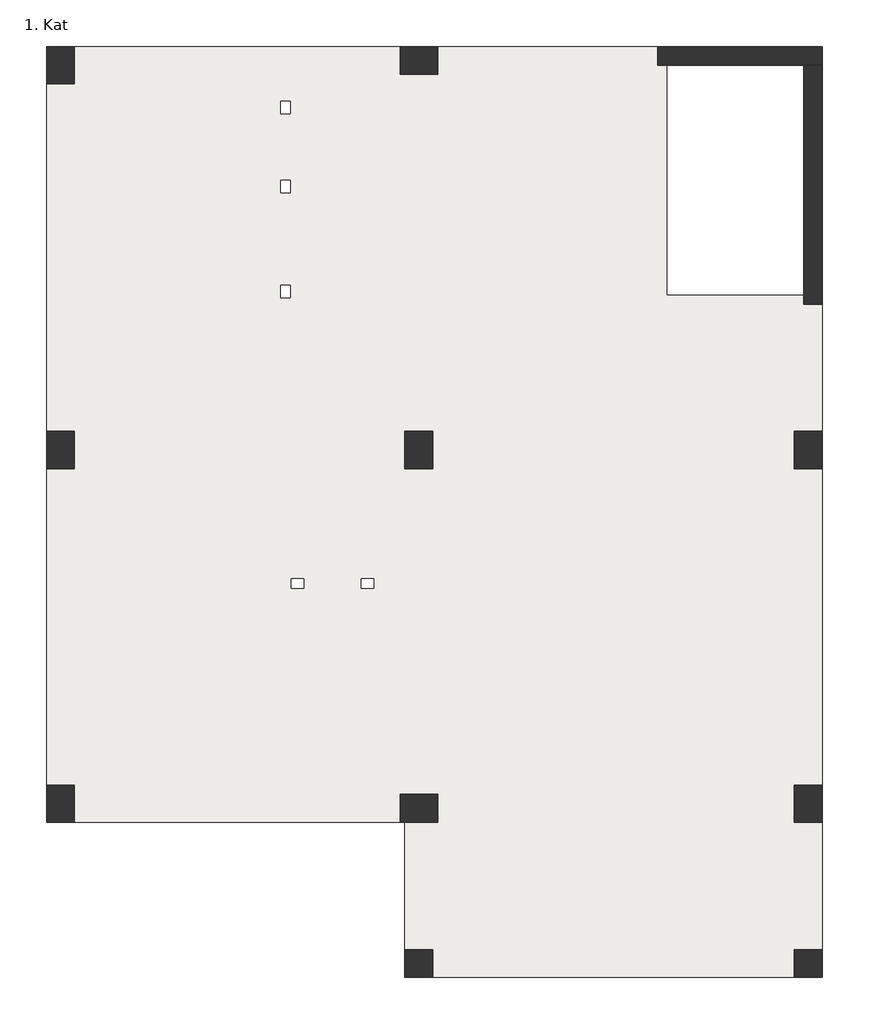
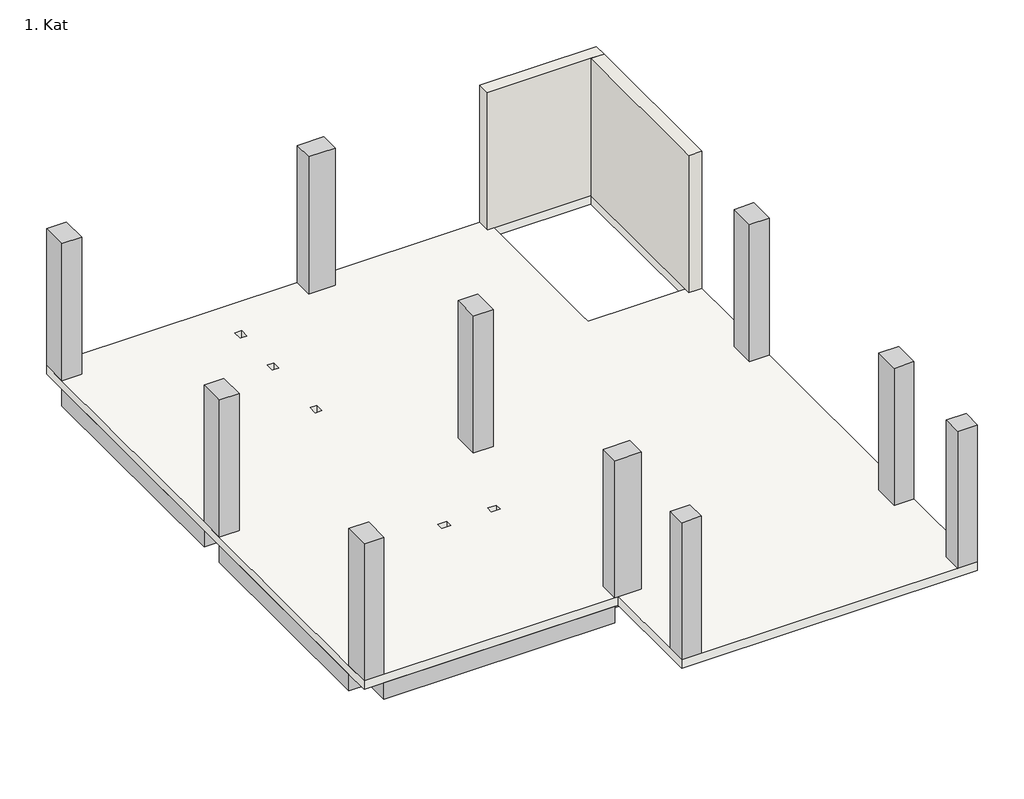
# One storey: 12 beams, 10 columns, 2 walls, 1 slab.
"""IFC4 building model written with IfcOpenShell, lengths in millimetres."""

from ifc_helpers import new_model, si_unit, frame, origin, place, context, project, spatial, polyline, outline, extrude, faceted_brep, element, save

model = new_model("IFC4")

# Units and contexts
model_context = context("Model", 3, world=origin())
ifc_project = project(units=[si_unit("LENGTHUNIT", "METRE", prefix="MILLI")], contexts=[model_context])

# Site, building, storey
site = spatial("IfcSite", under=ifc_project)
building = spatial("IfcBuilding", under=site)
storey = spatial("IfcBuildingStorey", under=building, Name="1. Kat", Elevation=97280.0)

# Beams
placement = place(None, origin())
element("IfcBeam", 1, ObjectType="M_Concrete-Rectangular Beam : 300 x 600mm", at=placement, inside=storey, context=model_context, shape_type="SweptSolid", body=[
    extrude(outline(polyline([(-8879.0485128, 8478.2904426), (-8879.0485128, 8778.2904426), (-5329.0485128, 8778.2904426), (-5329.0485128, 8478.2904426), (-8879.0485128, 8478.2904426)])), frame((0.0, 0.0, 96680.0), z_axis=(0.0, 0.0, 1.0), x_axis=(1.0, 0.0, 0.0)), (0.0, 0.0, 1.0), 400.0),
])
element("IfcBeam", 2, ObjectType="M_Concrete-Rectangular Beam : 300 x 600mm", at=placement, inside=storey, context=model_context, shape_type="SweptSolid", body=[
    extrude(outline(polyline([(-2679.0485128, 2578.2904426), (-2979.0485128, 2578.2904426), (-2979.0485128, 4628.2904426), (-2679.0485128, 4628.2904426), (-2679.0485128, 2578.2904426)])), frame((0.0, 0.0, 96680.0), z_axis=(0.0, 0.0, 1.0), x_axis=(1.0, 0.0, 0.0)), (0.0, 0.0, 1.0), 400.0),
])
element("IfcBeam", 3, ObjectType="M_Concrete-Rectangular Beam : 450 x 600mm", at=placement, inside=storey, context=model_context, shape_type="SweptSolid", body=[
    extrude(outline(polyline([(-8954.0485128, 1978.2904426), (-8954.0485128, -3271.7095574), (-9404.0485128, -3271.7095574), (-9404.0485128, 1978.2904426), (-8954.0485128, 1978.2904426)])), frame((0.0, 0.0, 96680.0), z_axis=(0.0, 0.0, 1.0), x_axis=(1.0, 0.0, 0.0)), (0.0, 0.0, 1.0), 400.0),
])
element("IfcBeam", 4, ObjectType="M_Concrete-Rectangular Beam : 450 x 600mm", at=placement, inside=storey, context=model_context, shape_type="SweptSolid", body=[
    extrude(outline(polyline([(-8954.0485128, 8328.2904426), (-8954.0485128, 2578.2904426), (-9404.0485128, 2578.2904426), (-9404.0485128, 8328.2904426), (-8954.0485128, 8328.2904426)])), frame((0.0, 0.0, 96680.0), z_axis=(0.0, 0.0, 1.0), x_axis=(1.0, 0.0, 0.0)), (0.0, 0.0, 1.0), 400.0),
])
element("IfcBeam", 5, ObjectType="M_Concrete-Rectangular Beam : 450 x 600mm", at=placement, inside=storey, context=model_context, shape_type="SweptSolid", body=[
    extrude(outline(polyline([(-9404.0485128, 2053.2904426), (-14729.0485128, 2053.2904426), (-14729.0485128, 2503.2904426), (-9404.0485128, 2503.2904426), (-9404.0485128, 2053.2904426)])), frame((0.0, 0.0, 96680.0), z_axis=(0.0, 0.0, 1.0), x_axis=(1.0, 0.0, 0.0)), (0.0, 0.0, 1.0), 400.0),
])
element("IfcBeam", 6, ObjectType="M_Concrete-Rectangular Beam : 450 x 600mm", at=placement, inside=storey, context=model_context, shape_type="SweptSolid", body=[
    extrude(outline(polyline([(-3129.0485128, 2053.2904426), (-8954.0485128, 2053.2904426), (-8954.0485128, 2503.2904426), (-3129.0485128, 2503.2904426), (-3129.0485128, 2053.2904426)])), frame((0.0, 0.0, 96680.0), z_axis=(0.0, 0.0, 1.0), x_axis=(1.0, 0.0, 0.0)), (0.0, 0.0, 1.0), 400.0),
])
element("IfcBeam", 7, ObjectType="M_Concrete-Rectangular Beam : 450 x 600mm", at=placement, inside=storey, context=model_context, shape_type="SweptSolid", body=[
    extrude(outline(polyline([(-9479.0485128, 8778.2904426), (-9479.0485128, 8328.2904426), (-14729.0485128, 8328.2904426), (-14729.0485128, 8778.2904426), (-9479.0485128, 8778.2904426)])), frame((0.0, 0.0, 96680.0), z_axis=(0.0, 0.0, 1.0), x_axis=(1.0, 0.0, 0.0)), (0.0, 0.0, 1.0), 400.0),
])
element("IfcBeam", 8, ObjectType="M_Concrete-Rectangular Beam : 450 x 600mm", at=placement, inside=storey, context=model_context, shape_type="SweptSolid", body=[
    extrude(outline(polyline([(-2679.0485128, -3121.7095574), (-3129.0485128, -3121.7095574), (-3129.0485128, 1978.2904426), (-2679.0485128, 1978.2904426), (-2679.0485128, -3121.7095574)])), frame((0.0, 0.0, 96680.0), z_axis=(0.0, 0.0, 1.0), x_axis=(1.0, 0.0, 0.0)), (0.0, 0.0, 1.0), 400.0),
])
element("IfcBeam", 9, ObjectType="M_Concrete-Rectangular Beam : 450 x 600mm", at=placement, inside=storey, context=model_context, shape_type="SweptSolid", body=[
    extrude(outline(polyline([(-9479.0485128, -3271.7095574), (-9479.0485128, -3721.7095574), (-14729.0485128, -3721.7095574), (-14729.0485128, -3271.7095574), (-9479.0485128, -3271.7095574)])), frame((0.0, 0.0, 96680.0), z_axis=(0.0, 0.0, 1.0), x_axis=(1.0, 0.0, 0.0)), (0.0, 0.0, 1.0), 400.0),
])
element("IfcBeam", 10, ObjectType="M_Concrete-Rectangular Beam : 450 x 600mm", at=placement, inside=storey, context=model_context, shape_type="SweptSolid", body=[
    extrude(outline(polyline([(-8879.0485128, -3721.7095574), (-8879.0485128, -3271.7095574), (-3129.0485128, -3271.7095574), (-3129.0485128, -3721.7095574), (-8879.0485128, -3721.7095574)])), frame((0.0, 0.0, 96680.0), z_axis=(0.0, 0.0, 1.0), x_axis=(1.0, 0.0, 0.0)), (0.0, 0.0, 1.0), 400.0),
])
element("IfcBeam", 11, ObjectType="M_Concrete-Rectangular Beam : 450 x 600mm", at=placement, inside=storey, context=model_context, shape_type="SweptSolid", body=[
    extrude(outline(polyline([(-14729.0485128, 2578.2904426), (-15179.0485128, 2578.2904426), (-15179.0485128, 8178.2904426), (-14729.0485128, 8178.2904426), (-14729.0485128, 2578.2904426)])), frame((0.0, 0.0, 96680.0), z_axis=(0.0, 0.0, 1.0), x_axis=(1.0, 0.0, 0.0)), (0.0, 0.0, 1.0), 400.0),
])
element("IfcBeam", 12, ObjectType="M_Concrete-Rectangular Beam : 450 x 600mm", at=placement, inside=storey, context=model_context, shape_type="SweptSolid", body=[
    extrude(outline(polyline([(-15179.0485128, 1978.2904426), (-14729.0485128, 1978.2904426), (-14729.0485128, -3121.7095574), (-15179.0485128, -3121.7095574), (-15179.0485128, 1978.2904426)])), frame((0.0, 0.0, 96680.0), z_axis=(0.0, 0.0, 1.0), x_axis=(1.0, 0.0, 0.0)), (0.0, 0.0, 1.0), 400.0),
])

# Columns
element("IfcColumn", 13, ObjectType="M_Concrete-Rectangular-Column : 450 x 450mm", at=placement, inside=storey, context=model_context, shape_type="SweptSolid", body=[
    extrude(outline(polyline([(-8954.0485128, -6221.7095574), (-9404.0485128, -6221.7095574), (-9404.0485128, -5771.7095574), (-8954.0485128, -5771.7095574), (-8954.0485128, -6221.7095574)])), frame((0.0, 0.0, 97280.0), z_axis=(0.0, 0.0, 1.0), x_axis=(1.0, 0.0, 0.0)), (0.0, 0.0, 1.0), 3300.0),
])
element("IfcColumn", 14, ObjectType="M_Concrete-Rectangular-Column : 450 x 450mm", at=placement, inside=storey, context=model_context, shape_type="SweptSolid", body=[
    extrude(outline(polyline([(-3129.0485128, -6221.7095574), (-3129.0485128, -5771.7095574), (-2679.0485128, -5771.7095574), (-2679.0485128, -6221.7095574), (-3129.0485128, -6221.7095574)])), frame((0.0, 0.0, 97280.0), z_axis=(0.0, 0.0, 1.0), x_axis=(1.0, 0.0, 0.0)), (0.0, 0.0, 1.0), 3300.0),
])
element("IfcColumn", 15, ObjectType="M_Concrete-Rectangular-Column : 450 x 600mm", at=placement, inside=storey, context=model_context, shape_type="SweptSolid", body=[
    extrude(outline(polyline([(-15179.0485128, -3721.7095574), (-15179.0485128, -3121.7095574), (-14729.0485128, -3121.7095574), (-14729.0485128, -3721.7095574), (-15179.0485128, -3721.7095574)])), frame((0.0, 0.0, 97280.0), z_axis=(0.0, 0.0, 1.0), x_axis=(1.0, 0.0, 0.0)), (0.0, 0.0, 1.0), 3300.0),
])
element("IfcColumn", 16, ObjectType="M_Concrete-Rectangular-Column : 450 x 600mm", at=placement, inside=storey, context=model_context, shape_type="SweptSolid", body=[
    extrude(outline(polyline([(-15179.0485128, 1978.2904426), (-15179.0485128, 2578.2904426), (-14729.0485128, 2578.2904426), (-14729.0485128, 1978.2904426), (-15179.0485128, 1978.2904426)])), frame((0.0, 0.0, 97280.0), z_axis=(0.0, 0.0, 1.0), x_axis=(1.0, 0.0, 0.0)), (0.0, 0.0, 1.0), 3300.0),
])
element("IfcColumn", 17, ObjectType="M_Concrete-Rectangular-Column : 450 x 600mm", at=placement, inside=storey, context=model_context, shape_type="SweptSolid", body=[
    extrude(outline(polyline([(-15179.0485128, 8178.2904426), (-15179.0485128, 8778.2904426), (-14729.0485128, 8778.2904426), (-14729.0485128, 8178.2904426), (-15179.0485128, 8178.2904426)])), frame((0.0, 0.0, 97280.0), z_axis=(0.0, 0.0, 1.0), x_axis=(1.0, 0.0, 0.0)), (0.0, 0.0, 1.0), 3300.0),
])
element("IfcColumn", 18, ObjectType="M_Concrete-Rectangular-Column : 450 x 600mm", at=placement, inside=storey, context=model_context, shape_type="Brep", body=[
    faceted_brep([(-8879.0485128, -3721.7095574, 97280.0), (-9404.0485128, -3721.7095574, 97280.0), (-9479.0485128, -3721.7095574, 97280.0), (-9479.0485128, -3271.7095574, 97280.0), (-8879.0485128, -3271.7095574, 97280.0), (-8879.0485128, -3721.7095574, 100580.0), (-9479.0485128, -3721.7095574, 100580.0), (-9479.0485128, -3271.7095574, 100580.0), (-8879.0485128, -3271.7095574, 100580.0)], [[[0, 1, 2, 3, 4]], [[2, 1, 0, 5, 6]], [[3, 2, 6, 7]], [[4, 3, 7, 8]], [[0, 4, 8, 5]], [[6, 5, 8, 7]]]),
])
element("IfcColumn", 19, ObjectType="M_Concrete-Rectangular-Column : 450 x 600mm", at=placement, inside=storey, context=model_context, shape_type="SweptSolid", body=[
    extrude(outline(polyline([(-9404.0485128, 1978.2904426), (-9404.0485128, 2578.2904426), (-8954.0485128, 2578.2904426), (-8954.0485128, 1978.2904426), (-9404.0485128, 1978.2904426)])), frame((0.0, 0.0, 97280.0), z_axis=(0.0, 0.0, 1.0), x_axis=(1.0, 0.0, 0.0)), (0.0, 0.0, 1.0), 3300.0),
])
element("IfcColumn", 20, ObjectType="M_Concrete-Rectangular-Column : 450 x 600mm", at=placement, inside=storey, context=model_context, shape_type="SweptSolid", body=[
    extrude(outline(polyline([(-8879.0485128, 8328.2904426), (-9479.0485128, 8328.2904426), (-9479.0485128, 8778.2904426), (-8879.0485128, 8778.2904426), (-8879.0485128, 8328.2904426)])), frame((0.0, 0.0, 97280.0), z_axis=(0.0, 0.0, 1.0), x_axis=(1.0, 0.0, 0.0)), (0.0, 0.0, 1.0), 3300.0),
])
element("IfcColumn", 21, ObjectType="M_Concrete-Rectangular-Column : 450 x 600mm", at=placement, inside=storey, context=model_context, shape_type="SweptSolid", body=[
    extrude(outline(polyline([(-3129.0485128, -3721.7095574), (-3129.0485128, -3121.7095574), (-2679.0485128, -3121.7095574), (-2679.0485128, -3721.7095574), (-3129.0485128, -3721.7095574)])), frame((0.0, 0.0, 97280.0), z_axis=(0.0, 0.0, 1.0), x_axis=(1.0, 0.0, 0.0)), (0.0, 0.0, 1.0), 3300.0),
])
element("IfcColumn", 22, ObjectType="M_Concrete-Rectangular-Column : 450 x 600mm", at=placement, inside=storey, context=model_context, shape_type="SweptSolid", body=[
    extrude(outline(polyline([(-3129.0485128, 1978.2904426), (-3129.0485128, 2578.2904426), (-2679.0485128, 2578.2904426), (-2679.0485128, 1978.2904426), (-3129.0485128, 1978.2904426)])), frame((0.0, 0.0, 97280.0), z_axis=(0.0, 0.0, 1.0), x_axis=(1.0, 0.0, 0.0)), (0.0, 0.0, 1.0), 3300.0),
])

# Slab
element("IfcSlab", 23, ObjectType="Generic 200mm", at=placement, inside=storey, context=model_context, shape_type="Brep", body=[
    faceted_brep([(-2679.0485128, 8778.2904426, 97080.0), (-2679.0485128, 4628.2904426, 97080.0), (-2679.0485128, 2578.2904426, 97080.0), (-2679.0485128, 1978.2904426, 97080.0), (-2679.0485128, -3121.7095574, 97080.0), (-2679.0485128, -3721.7095574, 97080.0), (-2679.0485128, -5771.7095574, 97080.0), (-2679.0485128, -6221.7095574, 97080.0), (-3129.0485128, -6221.7095574, 97080.0), (-8954.0485128, -6221.7095574, 97080.0), (-9404.0485128, -6221.7095574, 97080.0), (-9404.0485128, -5771.7095574, 97080.0), (-9404.0485128, -3721.7095574, 97080.0), (-9479.0485128, -3721.7095574, 97080.0), (-14729.0485128, -3721.7095574, 97080.0), (-15179.0485128, -3721.7095574, 97080.0), (-15179.0485128, -3121.7095574, 97080.0), (-15179.0485128, 1978.2904426, 97080.0), (-15179.0485128, 2578.2904426, 97080.0), (-15179.0485128, 8178.2904426, 97080.0), (-15179.0485128, 8778.2904426, 97080.0), (-14729.0485128, 8778.2904426, 97080.0), (-9479.0485128, 8778.2904426, 97080.0), (-8879.0485128, 8778.2904426, 97080.0), (-5329.0485128, 8778.2904426, 97080.0), (-2979.0485128, 4778.2904426, 97080.0), (-2979.0485128, 8478.2904426, 97080.0), (-5179.0485128, 8478.2904426, 97080.0), (-5179.0485128, 5253.2904426, 97080.0), (-5179.0485128, 5003.2904426, 97080.0), (-5179.0485128, 4778.2904426, 97080.0), (-4179.0485128, 4778.2904426, 97080.0), (-11404.0485128, 6624.8694152, 97080.0), (-11404.0485128, 6424.8694152, 97080.0), (-11254.0485128, 6424.8694152, 97080.0), (-11254.0485128, 6624.8694152, 97080.0), (-11404.0485128, 4933.2654426, 97080.0), (-11404.0485128, 4733.2654426, 97080.0), (-11254.0485128, 4733.2654426, 97080.0), (-11254.0485128, 4933.2654426, 97080.0), (-11404.0485128, 7898.2904426, 97080.0), (-11404.0485128, 7698.2904426, 97080.0), (-11254.0485128, 7698.2904426, 97080.0), (-11254.0485128, 7898.2904426, 97080.0), (-11232.3510299, 53.2904426, 97080.0), (-11032.3510299, 53.2904426, 97080.0), (-11032.3510299, 203.2904426, 97080.0), (-11232.3510299, 203.2904426, 97080.0), (-10104.0485128, 53.2904426, 97080.0), (-9904.0485128, 53.2904426, 97080.0), (-9904.0485128, 203.2904426, 97080.0), (-10104.0485128, 203.2904426, 97080.0), (-2679.0485128, -6221.7095574, 97280.0), (-2679.0485128, -5771.7095574, 97280.0), (-2679.0485128, -3721.7095574, 97280.0), (-2679.0485128, -3121.7095574, 97280.0), (-2679.0485128, 1978.2904426, 97280.0), (-2679.0485128, 2578.2904426, 97280.0), (-2679.0485128, 8778.2904426, 97280.0), (-8879.0485128, 8778.2904426, 97280.0), (-9479.0485128, 8778.2904426, 97280.0), (-14729.0485128, 8778.2904426, 97280.0), (-15179.0485128, 8778.2904426, 97280.0), (-15179.0485128, 8178.2904426, 97280.0), (-15179.0485128, 2578.2904426, 97280.0), (-15179.0485128, 1978.2904426, 97280.0), (-15179.0485128, -3121.7095574, 97280.0), (-15179.0485128, -3721.7095574, 97280.0), (-14729.0485128, -3721.7095574, 97280.0), (-9479.0485128, -3721.7095574, 97280.0), (-9404.0485128, -3721.7095574, 97280.0), (-9404.0485128, -5771.7095574, 97280.0), (-9404.0485128, -6221.7095574, 97280.0), (-8954.0485128, -6221.7095574, 97280.0), (-3129.0485128, -6221.7095574, 97280.0), (-2979.0485128, 8478.2904426, 97280.0), (-2979.0485128, 4778.2904426, 97280.0), (-4179.0485128, 4778.2904426, 97280.0), (-5179.0485128, 4778.2904426, 97280.0), (-5179.0485128, 5003.2904426, 97280.0), (-5179.0485128, 8478.2904426, 97280.0), (-11404.0485128, 6424.8694152, 97280.0), (-11404.0485128, 6624.8694152, 97280.0), (-11254.0485128, 6624.8694152, 97280.0), (-11254.0485128, 6424.8694152, 97280.0), (-11404.0485128, 4733.2654426, 97280.0), (-11404.0485128, 4933.2654426, 97280.0), (-11254.0485128, 4933.2654426, 97280.0), (-11254.0485128, 4733.2654426, 97280.0), (-11404.0485128, 7698.2904426, 97280.0), (-11404.0485128, 7898.2904426, 97280.0), (-11254.0485128, 7898.2904426, 97280.0), (-11254.0485128, 7698.2904426, 97280.0), (-11032.3510299, 53.2904426, 97280.0), (-11232.3510299, 53.2904426, 97280.0), (-11232.3510299, 203.2904426, 97280.0), (-11032.3510299, 203.2904426, 97280.0), (-9904.0485128, 53.2904426, 97280.0), (-10104.0485128, 53.2904426, 97280.0), (-10104.0485128, 203.2904426, 97280.0), (-9904.0485128, 203.2904426, 97280.0)], [[[0, 1, 2, 3, 4, 5, 6, 7, 8, 9, 10, 11, 12, 13, 14, 15, 16, 17, 18, 19, 20, 21, 22, 23, 24], [25, 26, 27, 28, 29, 30, 31], [32, 33, 34, 35], [36, 37, 38, 39], [40, 41, 42, 43], [44, 45, 46, 47], [48, 49, 50, 51]], [[52, 53, 54, 55, 56, 57, 58, 59, 60, 61, 62, 63, 64, 65, 66, 67, 68, 69, 70, 71, 72, 73, 74], [75, 76, 77, 78, 79, 80], [81, 82, 83, 84], [85, 86, 87, 88], [89, 90, 91, 92], [93, 94, 95, 96], [97, 98, 99, 100]], [[7, 6, 5, 4, 3, 2, 1, 0, 58, 57, 56, 55, 54, 53, 52]], [[15, 14, 13, 12, 70, 69, 68, 67]], [[20, 19, 18, 17, 16, 15, 67, 66, 65, 64, 63, 62]], [[0, 24, 23, 22, 21, 20, 62, 61, 60, 59, 58]], [[26, 25, 76, 75]], [[27, 26, 75, 80]], [[27, 80, 79, 78, 30, 29, 28]], [[30, 78, 77, 76, 25, 31]], [[10, 9, 8, 7, 52, 74, 73, 72]], [[12, 11, 10, 72, 71, 70]], [[32, 82, 81, 33]], [[33, 81, 84, 34]], [[34, 84, 83, 35]], [[82, 32, 35, 83]], [[36, 86, 85, 37]], [[37, 85, 88, 38]], [[38, 88, 87, 39]], [[86, 36, 39, 87]], [[40, 90, 89, 41]], [[41, 89, 92, 42]], [[42, 92, 91, 43]], [[90, 40, 43, 91]], [[44, 94, 93, 45]], [[45, 93, 96, 46]], [[46, 96, 95, 47]], [[94, 44, 47, 95]], [[48, 98, 97, 49]], [[49, 97, 100, 50]], [[50, 100, 99, 51]], [[98, 48, 51, 99]]]),
])

# Walls
element("IfcWall", 24, ObjectType="Generic - 300mm", at=placement, inside=storey, context=model_context, shape_type="Brep", body=[
    faceted_brep([(-2679.0485128, 8778.2904426, 97280.0), (-5329.0485128, 8778.2904426, 97280.0), (-5329.0485128, 8778.2904426, 100180.0), (-5329.0485128, 8778.2904426, 100580.0), (-2679.0485128, 8778.2904426, 100580.0), (-2679.0485128, 8478.2904426, 97280.0), (-2679.0485128, 8478.2904426, 100580.0), (-2979.0485128, 8478.2904426, 100580.0), (-5329.0485128, 8478.2904426, 100580.0), (-5329.0485128, 8478.2904426, 100180.0), (-5329.0485128, 8478.2904426, 97280.0), (-2979.0485128, 8478.2904426, 97280.0)], [[[0, 1, 2, 3, 4]], [[5, 6, 7, 8, 9, 10, 11]], [[1, 0, 5, 11, 10]], [[3, 2, 1, 10, 9, 8]], [[4, 3, 8, 7, 6]], [[0, 4, 6, 5]]]),
])
element("IfcWall", 25, ObjectType="Generic - 300mm", at=placement, inside=storey, context=model_context, shape_type="Brep", body=[
    faceted_brep([(-2979.0485128, 8478.2904426, 97280.0), (-2979.0485128, 4628.2904426, 97280.0), (-2979.0485128, 4628.2904426, 100180.0), (-2979.0485128, 4628.2904426, 100580.0), (-2979.0485128, 8478.2904426, 100580.0), (-2679.0485128, 8478.2904426, 97280.0), (-2679.0485128, 8478.2904426, 100580.0), (-2679.0485128, 4628.2904426, 100580.0), (-2679.0485128, 4628.2904426, 100180.0), (-2679.0485128, 4628.2904426, 97280.0)], [[[0, 1, 2, 3, 4]], [[5, 6, 7, 8, 9]], [[1, 0, 5, 9]], [[3, 2, 1, 9, 8, 7]], [[4, 3, 7, 6]], [[0, 4, 6, 5]]]),
])

save(model, "model.ifc")

# Revit data of these elements
# Type "M_Concrete-Rectangular Beam : 300 x 600mm"
#   Length [instance default] = 152.4 cm
#   b = 30 cm
#   h = 60 cm
#   Structural Material [instance default] = Concrete, Cast-in-Place gray
#   Assembly Code = ""
# Type "M_Concrete-Rectangular Beam : 450 x 600mm"
#   Length [instance default] = 152.4 cm
#   b = 45 cm
#   h = 60 cm
#   Structural Material [instance default] = Concrete, Cast-in-Place gray
#   Assembly Code = ""
# Type "M_Concrete-Rectangular-Column : 450 x 450mm"
#   b = 45 cm
#   h = 45 cm
#   Structural Material [instance default] = Concrete, Cast-in-Place gray
# Type "M_Concrete-Rectangular-Column : 450 x 600mm"
#   b = 45 cm
#   h = 60 cm
#   Structural Material [instance default] = Concrete, Cast-in-Place gray
# Type "Generic 200mm"
#   Function = 0
#   Layers, outside or top first: 20 cm "Concrete, Cast-in-Place gray" (function 1)
# Type "Generic - 300mm"
#   Layers, outside or top first: 30 cm "Concrete, Cast-in-Place gray" (function 1)
# Elements 1, 2 (IfcBeam, "M_Concrete-Rectangular Beam : 300 x 600mm")
#   Comments = ""
#   Structural Material = Concrete, Cast-in-Place gray
#   Phase Created = New Construction
#   Materials on its faces: "Concrete, Cast-in-Place gray"
# Elements 3, 4, 5, 6, 7, 8, 9, 10, 11, 12 (IfcBeam, "M_Concrete-Rectangular Beam : 450 x 600mm")
#   Comments = ""
#   Structural Material = Concrete, Cast-in-Place gray
#   Phase Created = New Construction
#   Materials on its faces: "Concrete, Cast-in-Place gray"
# Elements 13, 14 (IfcColumn, "M_Concrete-Rectangular-Column : 450 x 450mm")
#   Structural Material = Concrete, Cast-in-Place gray
#   Phase Created = New Construction
#   Materials on its faces: "Concrete, Cast-in-Place gray"
# Elements 15, 16, 17, 18, 19, 20, 21, 22 (IfcColumn, "M_Concrete-Rectangular-Column : 450 x 600mm")
#   Structural Material = Concrete, Cast-in-Place gray
#   Phase Created = New Construction
#   Materials on its faces: "Concrete, Cast-in-Place gray"
# Element 23 (IfcSlab, "Generic 200mm")
#   Height Offset From Level = 0 cm
#   built-in parameter 1001954 = 1
#   Phase Created = New Construction
#   Materials on its faces: "Concrete, Cast-in-Place gray"
# Elements 24, 25 (IfcWall, "Generic - 300mm")
#   Comments = ""
#   Top Offset = -20 cm
#   Base Offset = 0 cm
#   wall height = 330 cm
#   Phase Created = New Construction
#   Base Constraint = 1. Kat
#   Top Constraint = Çatı Katı
#   Materials on its faces: "Concrete, Cast-in-Place gray"
# Materials
#   "Concrete, Cast-in-Place gray": class "Concrete", colour RGB 192 192 192, transparency 0, Description = "Cast-in-place concrete", Cost = 0
